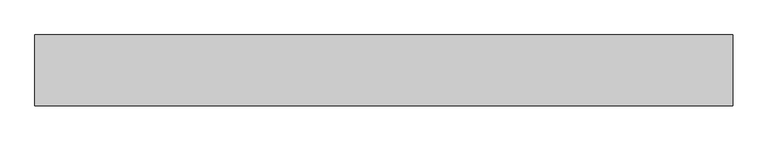
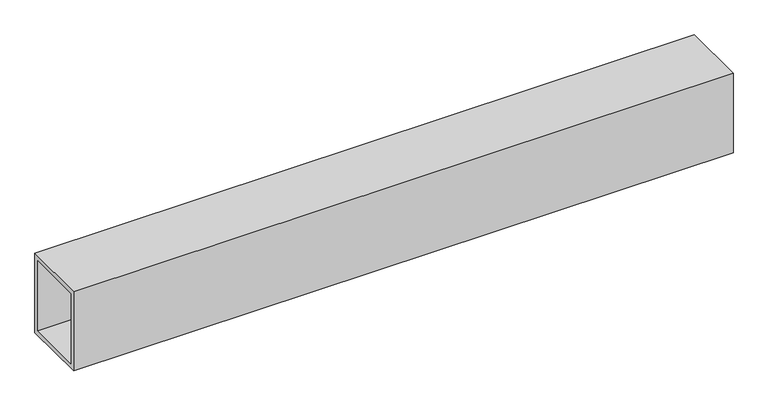
"""IFC4 building model written with IfcOpenShell, lengths in millimetres: proxy geometry, Structure060 11354 : Structure060 11354."""

import ifcopenshell
import ifcopenshell.guid

model = None  # the IFC model being written
_history = None  # IfcOwnerHistory: only IFC2X3 demands one
_inside = {}  # id of a spatial element -> (the spatial element, [elements in it])
_under = {}  # id of a project, library or spatial element -> (it, [spatial elements below it])
_declared = {}  # id of a project -> (the project, [libraries it declares])
_typed = {}  # id of a type object -> (the type object, [elements of that type])
_made_of = {}  # id of a material, layer set ... -> (it, [elements and type objects made of it])


def new_model(schema):
    """Start an empty IFC model of exactly this schema.

    Asked for "IFC4X3", IfcOpenShell would pick the latest addendum, in which some entities
    have other attributes; the version numbers below select the first issue.
    IFC2X3 requires an IfcOwnerHistory on every rooted entity: one is made here for all.
    """
    global model, _history
    if schema == "IFC4X3":
        model = ifcopenshell.file(schema_version=(4, 3, 0, 0))
    else:
        model = ifcopenshell.file(schema=schema)
    _inside.clear()
    _under.clear()
    _declared.clear()
    _typed.clear()
    _made_of.clear()
    _history = None
    if model.schema == "IFC2X3":
        org = make("IfcOrganization", Name="unknown")
        user = make(
            "IfcPersonAndOrganization",
            ThePerson=make("IfcPerson", FamilyName="unknown"),
            TheOrganization=org,
        )
        app = make(
            "IfcApplication",
            ApplicationDeveloper=org,
            Version="unknown",
            ApplicationFullName="unknown",
            ApplicationIdentifier="unknown",
        )
        _history = make(
            "IfcOwnerHistory",
            OwningUser=user,
            OwningApplication=app,
            ChangeAction="ADDED",
            CreationDate=0,
        )
    return model


def make(cls, **values):
    """One entity of the class cls with the attributes given. An attribute that is None is left unset."""
    return model.create_entity(
        cls, **{name: value for name, value in values.items() if value is not None}
    )


def rooted(cls, **values):
    """An entity with a GlobalId (a new one), such as an element, a storey or a relation."""
    return make(cls, GlobalId=ifcopenshell.guid.new(), OwnerHistory=_history, **values)


def si_unit(unit_type, name, prefix=None):
    """IfcSIUnit, for example si_unit("LENGTHUNIT", "METRE", prefix="MILLI")."""
    return make("IfcSIUnit", UnitType=unit_type, Prefix=prefix, Name=name)


def assignment(units):
    """IfcUnitAssignment: the units of a project."""
    return None if units is None else make("IfcUnitAssignment", Units=units)


def point(xyz):
    """IfcCartesianPoint."""
    return None if xyz is None else make("IfcCartesianPoint", Coordinates=xyz)


def direction(xyz):
    """IfcDirection."""
    return None if xyz is None else make("IfcDirection", DirectionRatios=xyz)


def frame(location, z_axis=None, x_axis=None):
    """IfcAxis2Placement3D, a coordinate frame: its origin and axes. An axis left out is left unset."""
    return make(
        "IfcAxis2Placement3D",
        Location=point(location),
        Axis=direction(z_axis),
        RefDirection=direction(x_axis),
    )


def origin():
    """The frame at (0, 0, 0) with its axes left unset."""
    return frame((0.0, 0.0, 0.0))


def place(relative_to, where):
    """IfcLocalPlacement: puts the frame where relative to a parent placement (None: the world)."""
    return make(
        "IfcLocalPlacement", PlacementRelTo=relative_to, RelativePlacement=where
    )


def context(
    kind, dimensions, precision=None, world=None, true_north=None, identifier=None
):
    """IfcGeometricRepresentationContext, for example the 3D "Model" context."""
    return make(
        "IfcGeometricRepresentationContext",
        ContextIdentifier=identifier,
        ContextType=kind,
        CoordinateSpaceDimension=dimensions,
        Precision=precision,
        WorldCoordinateSystem=world,
        TrueNorth=true_north,
    )


def project(units=None, contexts=None):
    """IfcProject with its units and contexts."""
    return rooted(
        "IfcProject",
        Name="project",
        RepresentationContexts=contexts,
        UnitsInContext=assignment(units),
    )


def spatial(cls, under=None, at=None, **own):
    """A site, building, storey or space (cls), placed at a placement, below another one or the project."""
    s = rooted(cls, ObjectPlacement=at, **own)
    if under is not None:
        _under.setdefault(under.id(), (under, []))[1].append(s)
    return s


def polyline(points):
    """IfcPolyline through the points."""
    return make("IfcPolyline", Points=[point(p) for p in points])


def outline(outer, holes=None, kind="AREA"):
    """IfcArbitraryClosedProfileDef: a profile drawn as a closed curve; with holes, ...WithVoids."""
    if holes is None:
        return make("IfcArbitraryClosedProfileDef", ProfileType=kind, OuterCurve=outer)
    return make(
        "IfcArbitraryProfileDefWithVoids",
        ProfileType=kind,
        OuterCurve=outer,
        InnerCurves=holes,
    )


def extrude(swept, where, along, depth):
    """IfcExtrudedAreaSolid: the profile swept, set in the frame where, extruded along a direction by depth."""
    return make(
        "IfcExtrudedAreaSolid",
        SweptArea=swept,
        Position=where,
        ExtrudedDirection=direction(along),
        Depth=depth,
    )


def shape(context_of_items, identifier, shape_type, items):
    """IfcShapeRepresentation: the items that make up one representation, for example the "Body"."""
    return make(
        "IfcShapeRepresentation",
        ContextOfItems=context_of_items,
        RepresentationIdentifier=identifier,
        RepresentationType=shape_type,
        Items=items,
    )


def source(mapping_origin, context_of_items, identifier, shape_type, items):
    """IfcRepresentationMap: a shape defined once, which mapped items show again and again."""
    return make(
        "IfcRepresentationMap",
        MappingOrigin=mapping_origin,
        MappedRepresentation=shape(context_of_items, identifier, shape_type, items),
    )


def transform(
    local_origin,
    x_axis=None,
    y_axis=None,
    z_axis=None,
    scale=None,
    scale2=None,
    scale3=None,
    uniform=True,
):
    """IfcCartesianTransformationOperator3D, or its non-uniform kind. x_axis, y_axis, z_axis: its Axis1, 2, 3."""
    if uniform:
        return make(
            "IfcCartesianTransformationOperator3D",
            Axis1=direction(x_axis),
            Axis2=direction(y_axis),
            LocalOrigin=point(local_origin),
            Scale=scale,
            Axis3=direction(z_axis),
        )
    return make(
        "IfcCartesianTransformationOperator3DnonUniform",
        Axis1=direction(x_axis),
        Axis2=direction(y_axis),
        LocalOrigin=point(local_origin),
        Scale=scale,
        Axis3=direction(z_axis),
        Scale2=scale2,
        Scale3=scale3,
    )


def mapped(mapping_source, mapping_target):
    """IfcMappedItem: shows the shape of a source again, moved by a transform."""
    return make(
        "IfcMappedItem", MappingSource=mapping_source, MappingTarget=mapping_target
    )


def made_of(thing, what):
    """Note that an element or type object is made of a material, layer set ...; save() writes the relation."""
    if what is not None:
        _made_of.setdefault(what.id(), (what, []))[1].append(thing)
    return thing


def element(
    cls,
    number,
    at=None,
    inside=None,
    cuts=None,
    type_object=None,
    material=None,
    context=None,
    identifier="Body",
    shape_type=None,
    held_by="IfcProductDefinitionShape",
    body=None,
    shapes=None,
    **own,
):
    """One element of the class cls, such as IfcWall. Its Tag is "e" and its number.

    at: its placement. inside: the storey or other place that contains it. cuts: it is an
    opening in that element (IfcRelVoidsElement). A single representation is given by context,
    identifier, shape_type and body (its items); several are given by shapes. held_by: the class
    of the entity that holds the representations. save() writes the other relations.
    """
    e = rooted(cls, Tag="e%d" % number, ObjectPlacement=at, **own)
    if body is not None:
        shapes = [shape(context, identifier, shape_type, body)]
    if shapes is not None:
        e.Representation = make(held_by, Representations=shapes)
    if inside is not None:
        _inside.setdefault(inside.id(), (inside, []))[1].append(e)
    if cuts is not None:
        rooted(
            "IfcRelVoidsElement", RelatingBuildingElement=cuts, RelatedOpeningElement=e
        )
    if type_object is not None:
        _typed.setdefault(type_object.id(), (type_object, []))[1].append(e)
    return made_of(e, material)


def aggregate(whole, parts):
    """IfcRelAggregates: a whole, such as a stair, and the parts it consists of."""
    return rooted("IfcRelAggregates", RelatingObject=whole, RelatedObjects=parts)


def save(model, path):
    """Write the relations noted so far, then the file.

    IfcRelAggregates (storeys below a building ...), IfcRelContainedInSpatialStructure (elements
    in a storey), IfcRelDefinesByType, IfcRelAssociatesMaterial and IfcRelDeclares: one each for
    every whole, place, type object, material and project.
    """
    for whole, parts in _under.values():
        aggregate(whole, parts)
    for where, things in _inside.values():
        rooted(
            "IfcRelContainedInSpatialStructure",
            RelatedElements=things,
            RelatingStructure=where,
        )
    for kind, things in _typed.values():
        rooted("IfcRelDefinesByType", RelatedObjects=things, RelatingType=kind)
    for what, things in _made_of.values():
        rooted("IfcRelAssociatesMaterial", RelatedObjects=things, RelatingMaterial=what)
    for by, libraries in _declared.values():
        rooted("IfcRelDeclares", RelatingContext=by, RelatedDefinitions=libraries)
    model.write(path)


def generic_models_8e027abe(model_context):
    return source(origin(), model_context, "Body", "SweptSolid", [
        extrude(outline(polyline([(2319.85766, 40087.2000712), (2319.85766, 39833.2000712), (2116.65766, 39833.2000712), (2116.65766, 40087.2000712), (2319.85766, 40087.2000712)]), holes=[polyline([(2305.1000924, 39847.9574608), (2305.1000924, 40072.4426608), (2131.4148924, 40072.4426608), (2131.4148924, 39847.9574608), (2305.1000924, 39847.9574608)])]), frame((6196.863802, 0.0, 0.0), z_axis=(1.0, 0.0, 0.0), x_axis=(0.0, 1.0, 0.0)), (0.0, 0.0, 1.0), 2000.0),
    ])


if __name__ == "__main__":
    model = new_model("IFC4")
    model_context = context("Model", 3, world=origin())
    ifc_project = project(units=[si_unit("LENGTHUNIT", "METRE", prefix="MILLI")], contexts=[model_context])
    site = spatial("IfcSite", under=ifc_project)
    building = spatial("IfcBuilding", under=site)
    placement = place(None, origin())
    generic_models_shape = generic_models_8e027abe(model_context)
    element("IfcBuildingElementProxy", 1, Name="Structure060 11354 : Structure060 11354", ObjectType="Structure060 11354 : Structure060 11354", at=placement, inside=building, context=model_context, shape_type="MappedRepresentation", body=[
        mapped(generic_models_shape, transform((0.0, 0.0, 0.0), x_axis=(1.0, 0.0, 0.0), y_axis=(0.0, 1.0, 0.0), z_axis=(0.0, 0.0, 1.0))),
    ])
    save(model, "model.ifc")

# Revit data of these elements
# Type "Structure060 11354 : Structure060 11354"
#   NameOverride = "Structure060"
# Element 1 (IfcBuildingElementProxy, "Structure060 11354 : Structure060 11354")
#   Materials on its faces: "STEEL STRUCTURE (SEE STRUCTURAL DWGS)"
# Materials
#   "STEEL STRUCTURE (SEE STRUCTURAL DWGS)": class "Unassigned", colour RGB 128 128 128, transparency 0, Cost = 0
